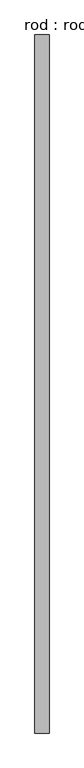
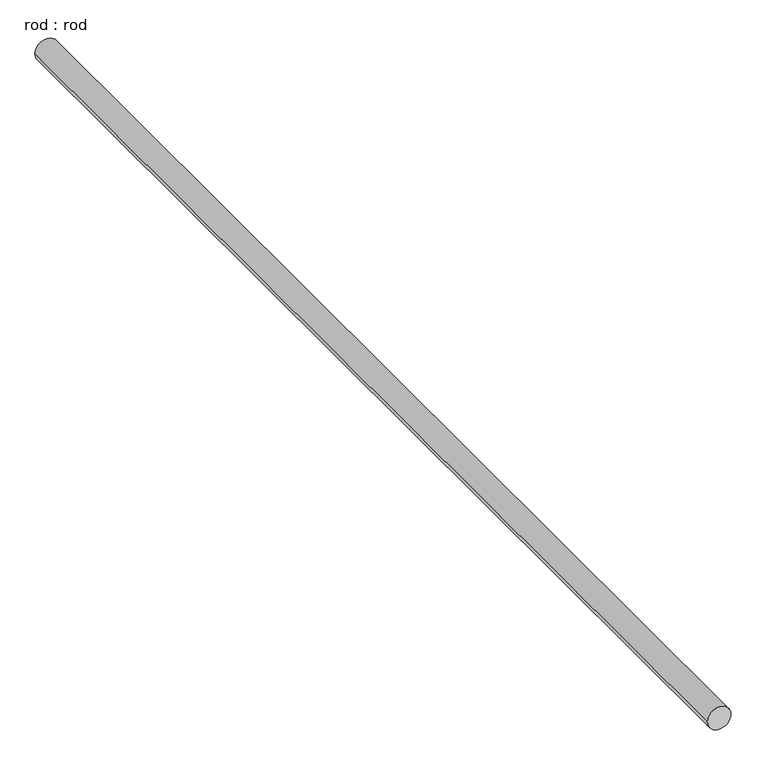
"""IFC4 building model written with IfcOpenShell, lengths in millimetres: proxy geometry, rod : rod."""

from ifc_helpers import new_model, si_unit, point, frame, frame_2d, origin, place, context, project, spatial, circle_curve, trimmed, segment, composite_curve, outline, extrude, source, transform, mapped, element, save


def rod_rod_964d58dc(model_context):
    return source(origin(), model_context, "Body", "SweptSolid", [
        extrude(outline(composite_curve([segment(trimmed(circle_curve(frame_2d((0.0108462, 0.0)), 200.0), [point((0.0108462, 200.0))], [point((0.0108462, -200.0))], False, "CARTESIAN"), True, "CONTINUOUS"), segment(trimmed(circle_curve(frame_2d((0.0108462, 0.0)), 200.0), [point((0.0108462, -200.0))], [point((0.0108462, 200.0))], False, "CARTESIAN"), True, "CONTINUOUS")], self_intersect=False)), frame((0.0, -5773.6475222, 0.0), z_axis=(0.0, 1.0, 0.0), x_axis=(0.0, 0.0, 1.0)), (0.0, 0.0, 1.0), 19732.752275),
    ])


if __name__ == "__main__":
    model = new_model("IFC4")
    model_context = context("Model", 3, world=origin())
    ifc_project = project(units=[si_unit("LENGTHUNIT", "METRE", prefix="MILLI")], contexts=[model_context])
    site = spatial("IfcSite", under=ifc_project)
    building = spatial("IfcBuilding", under=site)
    placement = place(None, origin())
    rod_rod_shape = rod_rod_964d58dc(model_context)
    element("IfcBuildingElementProxy", 1, Name="rod : rod", ObjectType="rod : rod", at=placement, inside=building, context=model_context, shape_type="MappedRepresentation", body=[
        mapped(rod_rod_shape, transform((0.0, 0.0, 0.0), x_axis=(1.0, 0.0, 0.0), y_axis=(0.0, 1.0, 0.0), z_axis=(0.0, 0.0, 1.0))),
    ])
    save(model, "model.ifc")

# Revit data of these elements
# Type "rod : rod"
#   Default Elevation = 0
